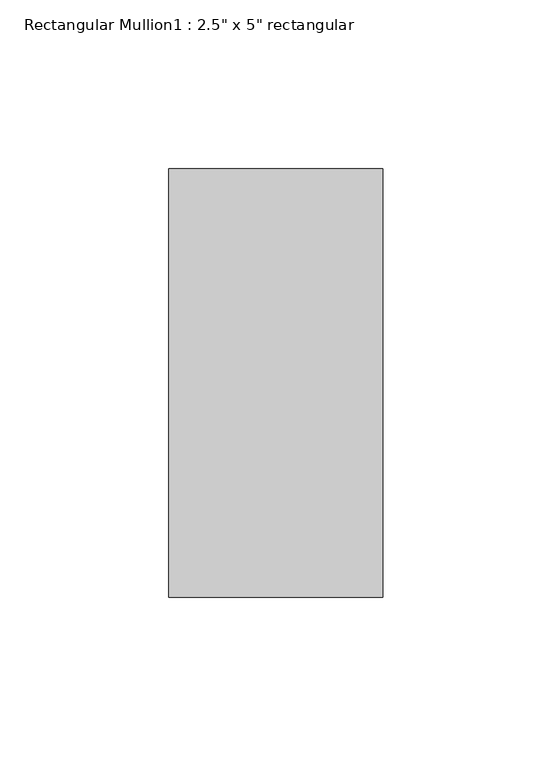
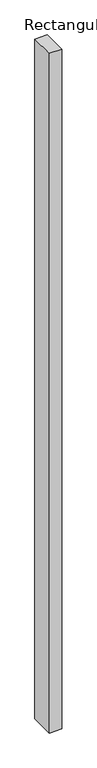
"""IFC4 building model written with IfcOpenShell, lengths in millimetres: member geometry."""

import ifcopenshell
import ifcopenshell.guid

model = None  # the IFC model being written
_history = None  # IfcOwnerHistory: only IFC2X3 demands one
_inside = {}  # id of a spatial element -> (the spatial element, [elements in it])
_under = {}  # id of a project, library or spatial element -> (it, [spatial elements below it])
_declared = {}  # id of a project -> (the project, [libraries it declares])
_typed = {}  # id of a type object -> (the type object, [elements of that type])
_made_of = {}  # id of a material, layer set ... -> (it, [elements and type objects made of it])


def new_model(schema):
    """Start an empty IFC model of exactly this schema.

    Asked for "IFC4X3", IfcOpenShell would pick the latest addendum, in which some entities
    have other attributes; the version numbers below select the first issue.
    IFC2X3 requires an IfcOwnerHistory on every rooted entity: one is made here for all.
    """
    global model, _history
    if schema == "IFC4X3":
        model = ifcopenshell.file(schema_version=(4, 3, 0, 0))
    else:
        model = ifcopenshell.file(schema=schema)
    _inside.clear()
    _under.clear()
    _declared.clear()
    _typed.clear()
    _made_of.clear()
    _history = None
    if model.schema == "IFC2X3":
        org = make("IfcOrganization", Name="unknown")
        user = make(
            "IfcPersonAndOrganization",
            ThePerson=make("IfcPerson", FamilyName="unknown"),
            TheOrganization=org,
        )
        app = make(
            "IfcApplication",
            ApplicationDeveloper=org,
            Version="unknown",
            ApplicationFullName="unknown",
            ApplicationIdentifier="unknown",
        )
        _history = make(
            "IfcOwnerHistory",
            OwningUser=user,
            OwningApplication=app,
            ChangeAction="ADDED",
            CreationDate=0,
        )
    return model


def make(cls, **values):
    """One entity of the class cls with the attributes given. An attribute that is None is left unset."""
    return model.create_entity(
        cls, **{name: value for name, value in values.items() if value is not None}
    )


def rooted(cls, **values):
    """An entity with a GlobalId (a new one), such as an element, a storey or a relation."""
    return make(cls, GlobalId=ifcopenshell.guid.new(), OwnerHistory=_history, **values)


def si_unit(unit_type, name, prefix=None):
    """IfcSIUnit, for example si_unit("LENGTHUNIT", "METRE", prefix="MILLI")."""
    return make("IfcSIUnit", UnitType=unit_type, Prefix=prefix, Name=name)


def assignment(units):
    """IfcUnitAssignment: the units of a project."""
    return None if units is None else make("IfcUnitAssignment", Units=units)


def point(xyz):
    """IfcCartesianPoint."""
    return None if xyz is None else make("IfcCartesianPoint", Coordinates=xyz)


def direction(xyz):
    """IfcDirection."""
    return None if xyz is None else make("IfcDirection", DirectionRatios=xyz)


def frame(location, z_axis=None, x_axis=None):
    """IfcAxis2Placement3D, a coordinate frame: its origin and axes. An axis left out is left unset."""
    return make(
        "IfcAxis2Placement3D",
        Location=point(location),
        Axis=direction(z_axis),
        RefDirection=direction(x_axis),
    )


def origin():
    """The frame at (0, 0, 0) with its axes left unset."""
    return frame((0.0, 0.0, 0.0))


def place(relative_to, where):
    """IfcLocalPlacement: puts the frame where relative to a parent placement (None: the world)."""
    return make(
        "IfcLocalPlacement", PlacementRelTo=relative_to, RelativePlacement=where
    )


def context(
    kind, dimensions, precision=None, world=None, true_north=None, identifier=None
):
    """IfcGeometricRepresentationContext, for example the 3D "Model" context."""
    return make(
        "IfcGeometricRepresentationContext",
        ContextIdentifier=identifier,
        ContextType=kind,
        CoordinateSpaceDimension=dimensions,
        Precision=precision,
        WorldCoordinateSystem=world,
        TrueNorth=true_north,
    )


def project(units=None, contexts=None):
    """IfcProject with its units and contexts."""
    return rooted(
        "IfcProject",
        Name="project",
        RepresentationContexts=contexts,
        UnitsInContext=assignment(units),
    )


def spatial(cls, under=None, at=None, **own):
    """A site, building, storey or space (cls), placed at a placement, below another one or the project."""
    s = rooted(cls, ObjectPlacement=at, **own)
    if under is not None:
        _under.setdefault(under.id(), (under, []))[1].append(s)
    return s


def polyline(points):
    """IfcPolyline through the points."""
    return make("IfcPolyline", Points=[point(p) for p in points])


def outline(outer, holes=None, kind="AREA"):
    """IfcArbitraryClosedProfileDef: a profile drawn as a closed curve; with holes, ...WithVoids."""
    if holes is None:
        return make("IfcArbitraryClosedProfileDef", ProfileType=kind, OuterCurve=outer)
    return make(
        "IfcArbitraryProfileDefWithVoids",
        ProfileType=kind,
        OuterCurve=outer,
        InnerCurves=holes,
    )


def extrude(swept, where, along, depth):
    """IfcExtrudedAreaSolid: the profile swept, set in the frame where, extruded along a direction by depth."""
    return make(
        "IfcExtrudedAreaSolid",
        SweptArea=swept,
        Position=where,
        ExtrudedDirection=direction(along),
        Depth=depth,
    )


def shape(context_of_items, identifier, shape_type, items):
    """IfcShapeRepresentation: the items that make up one representation, for example the "Body"."""
    return make(
        "IfcShapeRepresentation",
        ContextOfItems=context_of_items,
        RepresentationIdentifier=identifier,
        RepresentationType=shape_type,
        Items=items,
    )


def source(mapping_origin, context_of_items, identifier, shape_type, items):
    """IfcRepresentationMap: a shape defined once, which mapped items show again and again."""
    return make(
        "IfcRepresentationMap",
        MappingOrigin=mapping_origin,
        MappedRepresentation=shape(context_of_items, identifier, shape_type, items),
    )


def transform(
    local_origin,
    x_axis=None,
    y_axis=None,
    z_axis=None,
    scale=None,
    scale2=None,
    scale3=None,
    uniform=True,
):
    """IfcCartesianTransformationOperator3D, or its non-uniform kind. x_axis, y_axis, z_axis: its Axis1, 2, 3."""
    if uniform:
        return make(
            "IfcCartesianTransformationOperator3D",
            Axis1=direction(x_axis),
            Axis2=direction(y_axis),
            LocalOrigin=point(local_origin),
            Scale=scale,
            Axis3=direction(z_axis),
        )
    return make(
        "IfcCartesianTransformationOperator3DnonUniform",
        Axis1=direction(x_axis),
        Axis2=direction(y_axis),
        LocalOrigin=point(local_origin),
        Scale=scale,
        Axis3=direction(z_axis),
        Scale2=scale2,
        Scale3=scale3,
    )


def mapped(mapping_source, mapping_target):
    """IfcMappedItem: shows the shape of a source again, moved by a transform."""
    return make(
        "IfcMappedItem", MappingSource=mapping_source, MappingTarget=mapping_target
    )


def made_of(thing, what):
    """Note that an element or type object is made of a material, layer set ...; save() writes the relation."""
    if what is not None:
        _made_of.setdefault(what.id(), (what, []))[1].append(thing)
    return thing


def element(
    cls,
    number,
    at=None,
    inside=None,
    cuts=None,
    type_object=None,
    material=None,
    context=None,
    identifier="Body",
    shape_type=None,
    held_by="IfcProductDefinitionShape",
    body=None,
    shapes=None,
    **own,
):
    """One element of the class cls, such as IfcWall. Its Tag is "e" and its number.

    at: its placement. inside: the storey or other place that contains it. cuts: it is an
    opening in that element (IfcRelVoidsElement). A single representation is given by context,
    identifier, shape_type and body (its items); several are given by shapes. held_by: the class
    of the entity that holds the representations. save() writes the other relations.
    """
    e = rooted(cls, Tag="e%d" % number, ObjectPlacement=at, **own)
    if body is not None:
        shapes = [shape(context, identifier, shape_type, body)]
    if shapes is not None:
        e.Representation = make(held_by, Representations=shapes)
    if inside is not None:
        _inside.setdefault(inside.id(), (inside, []))[1].append(e)
    if cuts is not None:
        rooted(
            "IfcRelVoidsElement", RelatingBuildingElement=cuts, RelatedOpeningElement=e
        )
    if type_object is not None:
        _typed.setdefault(type_object.id(), (type_object, []))[1].append(e)
    return made_of(e, material)


def aggregate(whole, parts):
    """IfcRelAggregates: a whole, such as a stair, and the parts it consists of."""
    return rooted("IfcRelAggregates", RelatingObject=whole, RelatedObjects=parts)


def save(model, path):
    """Write the relations noted so far, then the file.

    IfcRelAggregates (storeys below a building ...), IfcRelContainedInSpatialStructure (elements
    in a storey), IfcRelDefinesByType, IfcRelAssociatesMaterial and IfcRelDeclares: one each for
    every whole, place, type object, material and project.
    """
    for whole, parts in _under.values():
        aggregate(whole, parts)
    for where, things in _inside.values():
        rooted(
            "IfcRelContainedInSpatialStructure",
            RelatedElements=things,
            RelatingStructure=where,
        )
    for kind, things in _typed.values():
        rooted("IfcRelDefinesByType", RelatedObjects=things, RelatingType=kind)
    for what, things in _made_of.values():
        rooted("IfcRelAssociatesMaterial", RelatedObjects=things, RelatingMaterial=what)
    for by, libraries in _declared.values():
        rooted("IfcRelDeclares", RelatingContext=by, RelatedDefinitions=libraries)
    model.write(path)


def member_4d31274b(model_context):
    return source(origin(), model_context, "Body", "SweptSolid", [
        extrude(outline(polyline([(0.0, 63.5), (0.0, -63.5), (-63.5, -63.5), (-63.5, 63.5), (0.0, 63.5)])), frame((0.0, 0.0, -3657.6), z_axis=(0.0, 0.0, 1.0), x_axis=(1.0, 0.0, 0.0)), (0.0, 0.0, 1.0), 3657.6),
    ])


if __name__ == "__main__":
    model = new_model("IFC4")
    model_context = context("Model", 3, world=origin())
    ifc_project = project(units=[si_unit("LENGTHUNIT", "METRE", prefix="MILLI")], contexts=[model_context])
    site = spatial("IfcSite", under=ifc_project)
    building = spatial("IfcBuilding", under=site)
    placement = place(None, origin())
    member_shape = member_4d31274b(model_context)
    element("IfcMember", 1, ObjectType="Rectangular Mullion1 : 2.5\" x 5\" rectangular", at=placement, inside=building, context=model_context, shape_type="MappedRepresentation", body=[
        mapped(member_shape, transform((0.0, 0.0, 0.0), x_axis=(1.0, 0.0, 0.0), y_axis=(0.0, 1.0, 0.0), z_axis=(0.0, 0.0, 1.0))),
    ])
    save(model, "model.ifc")

# Revit data of these elements
# Type "Rectangular Mullion1 : 2.5\" x 5\" rectangular"
#   built-in parameter 1007304 = 0.416667 (stored number, unit not read)
#   built-in parameter 1007301 = 0.104167 (stored number, unit not read)
#   built-in parameter 1007300 = 0.104167 (stored number, unit not read)
# Element 1 (IfcMember, "Rectangular Mullion1 : 2.5\" x 5\" rectangular")
#   Materials on its faces: "support-frame"
# Materials
#   "support-frame": class "Unassigned", colour RGB 233 233 233, transparency 0, Cost = 0
